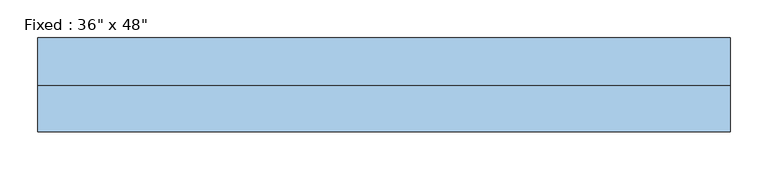
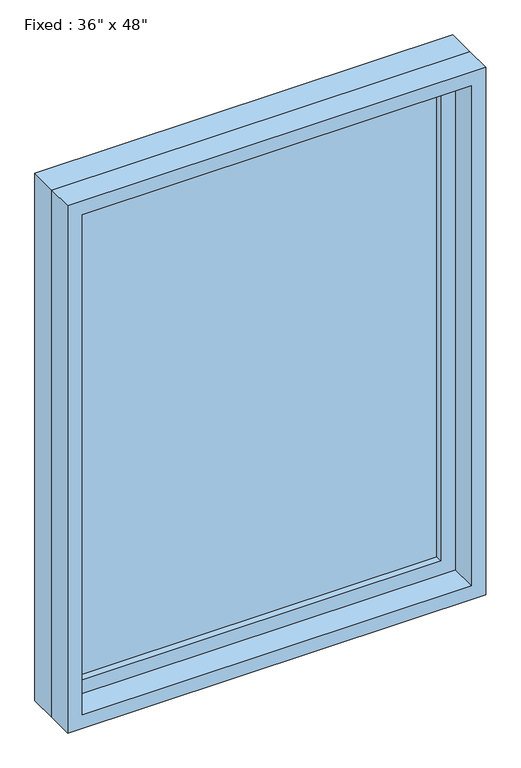
"""IFC4 building model written with IfcOpenShell, lengths in millimetres: window geometry."""

import ifcopenshell
import ifcopenshell.guid

model = None  # the IFC model being written
_history = None  # IfcOwnerHistory: only IFC2X3 demands one
_inside = {}  # id of a spatial element -> (the spatial element, [elements in it])
_under = {}  # id of a project, library or spatial element -> (it, [spatial elements below it])
_declared = {}  # id of a project -> (the project, [libraries it declares])
_typed = {}  # id of a type object -> (the type object, [elements of that type])
_made_of = {}  # id of a material, layer set ... -> (it, [elements and type objects made of it])


def new_model(schema):
    """Start an empty IFC model of exactly this schema.

    Asked for "IFC4X3", IfcOpenShell would pick the latest addendum, in which some entities
    have other attributes; the version numbers below select the first issue.
    IFC2X3 requires an IfcOwnerHistory on every rooted entity: one is made here for all.
    """
    global model, _history
    if schema == "IFC4X3":
        model = ifcopenshell.file(schema_version=(4, 3, 0, 0))
    else:
        model = ifcopenshell.file(schema=schema)
    _inside.clear()
    _under.clear()
    _declared.clear()
    _typed.clear()
    _made_of.clear()
    _history = None
    if model.schema == "IFC2X3":
        org = make("IfcOrganization", Name="unknown")
        user = make(
            "IfcPersonAndOrganization",
            ThePerson=make("IfcPerson", FamilyName="unknown"),
            TheOrganization=org,
        )
        app = make(
            "IfcApplication",
            ApplicationDeveloper=org,
            Version="unknown",
            ApplicationFullName="unknown",
            ApplicationIdentifier="unknown",
        )
        _history = make(
            "IfcOwnerHistory",
            OwningUser=user,
            OwningApplication=app,
            ChangeAction="ADDED",
            CreationDate=0,
        )
    return model


def make(cls, **values):
    """One entity of the class cls with the attributes given. An attribute that is None is left unset."""
    return model.create_entity(
        cls, **{name: value for name, value in values.items() if value is not None}
    )


def rooted(cls, **values):
    """An entity with a GlobalId (a new one), such as an element, a storey or a relation."""
    return make(cls, GlobalId=ifcopenshell.guid.new(), OwnerHistory=_history, **values)


def si_unit(unit_type, name, prefix=None):
    """IfcSIUnit, for example si_unit("LENGTHUNIT", "METRE", prefix="MILLI")."""
    return make("IfcSIUnit", UnitType=unit_type, Prefix=prefix, Name=name)


def assignment(units):
    """IfcUnitAssignment: the units of a project."""
    return None if units is None else make("IfcUnitAssignment", Units=units)


def point(xyz):
    """IfcCartesianPoint."""
    return None if xyz is None else make("IfcCartesianPoint", Coordinates=xyz)


def direction(xyz):
    """IfcDirection."""
    return None if xyz is None else make("IfcDirection", DirectionRatios=xyz)


def frame(location, z_axis=None, x_axis=None):
    """IfcAxis2Placement3D, a coordinate frame: its origin and axes. An axis left out is left unset."""
    return make(
        "IfcAxis2Placement3D",
        Location=point(location),
        Axis=direction(z_axis),
        RefDirection=direction(x_axis),
    )


def origin():
    """The frame at (0, 0, 0) with its axes left unset."""
    return frame((0.0, 0.0, 0.0))


def place(relative_to, where):
    """IfcLocalPlacement: puts the frame where relative to a parent placement (None: the world)."""
    return make(
        "IfcLocalPlacement", PlacementRelTo=relative_to, RelativePlacement=where
    )


def context(
    kind, dimensions, precision=None, world=None, true_north=None, identifier=None
):
    """IfcGeometricRepresentationContext, for example the 3D "Model" context."""
    return make(
        "IfcGeometricRepresentationContext",
        ContextIdentifier=identifier,
        ContextType=kind,
        CoordinateSpaceDimension=dimensions,
        Precision=precision,
        WorldCoordinateSystem=world,
        TrueNorth=true_north,
    )


def project(units=None, contexts=None):
    """IfcProject with its units and contexts."""
    return rooted(
        "IfcProject",
        Name="project",
        RepresentationContexts=contexts,
        UnitsInContext=assignment(units),
    )


def spatial(cls, under=None, at=None, **own):
    """A site, building, storey or space (cls), placed at a placement, below another one or the project."""
    s = rooted(cls, ObjectPlacement=at, **own)
    if under is not None:
        _under.setdefault(under.id(), (under, []))[1].append(s)
    return s


def polyline(points):
    """IfcPolyline through the points."""
    return make("IfcPolyline", Points=[point(p) for p in points])


def outline(outer, holes=None, kind="AREA"):
    """IfcArbitraryClosedProfileDef: a profile drawn as a closed curve; with holes, ...WithVoids."""
    if holes is None:
        return make("IfcArbitraryClosedProfileDef", ProfileType=kind, OuterCurve=outer)
    return make(
        "IfcArbitraryProfileDefWithVoids",
        ProfileType=kind,
        OuterCurve=outer,
        InnerCurves=holes,
    )


def extrude(swept, where, along, depth):
    """IfcExtrudedAreaSolid: the profile swept, set in the frame where, extruded along a direction by depth."""
    return make(
        "IfcExtrudedAreaSolid",
        SweptArea=swept,
        Position=where,
        ExtrudedDirection=direction(along),
        Depth=depth,
    )


def shape(context_of_items, identifier, shape_type, items):
    """IfcShapeRepresentation: the items that make up one representation, for example the "Body"."""
    return make(
        "IfcShapeRepresentation",
        ContextOfItems=context_of_items,
        RepresentationIdentifier=identifier,
        RepresentationType=shape_type,
        Items=items,
    )


def source(mapping_origin, context_of_items, identifier, shape_type, items):
    """IfcRepresentationMap: a shape defined once, which mapped items show again and again."""
    return make(
        "IfcRepresentationMap",
        MappingOrigin=mapping_origin,
        MappedRepresentation=shape(context_of_items, identifier, shape_type, items),
    )


def transform(
    local_origin,
    x_axis=None,
    y_axis=None,
    z_axis=None,
    scale=None,
    scale2=None,
    scale3=None,
    uniform=True,
):
    """IfcCartesianTransformationOperator3D, or its non-uniform kind. x_axis, y_axis, z_axis: its Axis1, 2, 3."""
    if uniform:
        return make(
            "IfcCartesianTransformationOperator3D",
            Axis1=direction(x_axis),
            Axis2=direction(y_axis),
            LocalOrigin=point(local_origin),
            Scale=scale,
            Axis3=direction(z_axis),
        )
    return make(
        "IfcCartesianTransformationOperator3DnonUniform",
        Axis1=direction(x_axis),
        Axis2=direction(y_axis),
        LocalOrigin=point(local_origin),
        Scale=scale,
        Axis3=direction(z_axis),
        Scale2=scale2,
        Scale3=scale3,
    )


def mapped(mapping_source, mapping_target):
    """IfcMappedItem: shows the shape of a source again, moved by a transform."""
    return make(
        "IfcMappedItem", MappingSource=mapping_source, MappingTarget=mapping_target
    )


def made_of(thing, what):
    """Note that an element or type object is made of a material, layer set ...; save() writes the relation."""
    if what is not None:
        _made_of.setdefault(what.id(), (what, []))[1].append(thing)
    return thing


def element(
    cls,
    number,
    at=None,
    inside=None,
    cuts=None,
    type_object=None,
    material=None,
    context=None,
    identifier="Body",
    shape_type=None,
    held_by="IfcProductDefinitionShape",
    body=None,
    shapes=None,
    **own,
):
    """One element of the class cls, such as IfcWall. Its Tag is "e" and its number.

    at: its placement. inside: the storey or other place that contains it. cuts: it is an
    opening in that element (IfcRelVoidsElement). A single representation is given by context,
    identifier, shape_type and body (its items); several are given by shapes. held_by: the class
    of the entity that holds the representations. save() writes the other relations.
    """
    e = rooted(cls, Tag="e%d" % number, ObjectPlacement=at, **own)
    if body is not None:
        shapes = [shape(context, identifier, shape_type, body)]
    if shapes is not None:
        e.Representation = make(held_by, Representations=shapes)
    if inside is not None:
        _inside.setdefault(inside.id(), (inside, []))[1].append(e)
    if cuts is not None:
        rooted(
            "IfcRelVoidsElement", RelatingBuildingElement=cuts, RelatedOpeningElement=e
        )
    if type_object is not None:
        _typed.setdefault(type_object.id(), (type_object, []))[1].append(e)
    return made_of(e, material)


def aggregate(whole, parts):
    """IfcRelAggregates: a whole, such as a stair, and the parts it consists of."""
    return rooted("IfcRelAggregates", RelatingObject=whole, RelatedObjects=parts)


def save(model, path):
    """Write the relations noted so far, then the file.

    IfcRelAggregates (storeys below a building ...), IfcRelContainedInSpatialStructure (elements
    in a storey), IfcRelDefinesByType, IfcRelAssociatesMaterial and IfcRelDeclares: one each for
    every whole, place, type object, material and project.
    """
    for whole, parts in _under.values():
        aggregate(whole, parts)
    for where, things in _inside.values():
        rooted(
            "IfcRelContainedInSpatialStructure",
            RelatedElements=things,
            RelatingStructure=where,
        )
    for kind, things in _typed.values():
        rooted("IfcRelDefinesByType", RelatedObjects=things, RelatingType=kind)
    for what, things in _made_of.values():
        rooted("IfcRelAssociatesMaterial", RelatedObjects=things, RelatingMaterial=what)
    for by, libraries in _declared.values():
        rooted("IfcRelDeclares", RelatingContext=by, RelatedDefinitions=libraries)
    model.write(path)


def window_96cf1632(model_context):
    return source(origin(), model_context, "Body", "SweptSolid", [
        extrude(outline(polyline([(355.6, 14.2875), (-431.8, 14.2875), (-431.8, 26.9875), (355.6, 26.9875), (355.6, 14.2875)])), frame((0.0, 0.0, 977.9), z_axis=(0.0, 0.0, 1.0), x_axis=(1.0, 0.0, 0.0)), (0.0, 0.0, 1.0), 1092.2),
        extrude(outline(polyline([(2114.55, -476.25), (933.45, -476.25), (933.45, 400.05), (2114.55, 400.05), (2114.55, -476.25)]), holes=[polyline([(2070.1, -431.8), (2070.1, 355.6), (977.9, 355.6), (977.9, -431.8), (2070.1, -431.8)])]), frame((0.0, -1.5875, 0.0), z_axis=(0.0, 1.0, 0.0), x_axis=(0.0, 0.0, 1.0)), (0.0, 0.0, 1.0), 44.45),
        extrude(outline(polyline([(2133.6, -495.3), (914.4, -495.3), (914.4, 419.1), (2133.6, 419.1), (2133.6, -495.3)]), holes=[polyline([(2101.85, -463.55), (2101.85, 387.35), (946.15, 387.35), (946.15, -463.55), (2101.85, -463.55)])]), frame((0.0, -61.9125, 0.0), z_axis=(0.0, 1.0, 0.0), x_axis=(0.0, 0.0, 1.0)), (0.0, 0.0, 1.0), 60.325),
        extrude(outline(polyline([(2133.6, 419.1), (2133.6, -495.3), (914.4, -495.3), (914.4, 419.1), (2133.6, 419.1)]), holes=[polyline([(2114.55, 400.05), (933.45, 400.05), (933.45, -476.25), (2114.55, -476.25), (2114.55, 400.05)])]), frame((0.0, -1.5875, 0.0), z_axis=(0.0, 1.0, 0.0), x_axis=(0.0, 0.0, 1.0)), (0.0, 0.0, 1.0), 63.5),
    ])


if __name__ == "__main__":
    model = new_model("IFC4")
    model_context = context("Model", 3, world=origin())
    ifc_project = project(units=[si_unit("LENGTHUNIT", "METRE", prefix="MILLI")], contexts=[model_context])
    site = spatial("IfcSite", under=ifc_project)
    building = spatial("IfcBuilding", under=site)
    placement = place(None, origin())
    window_shape = window_96cf1632(model_context)
    element("IfcWindow", 1, ObjectType="Fixed : 36\" x 48\"", at=placement, inside=building, context=model_context, shape_type="MappedRepresentation", body=[
        mapped(window_shape, transform((0.0, 0.0, 0.0), x_axis=(1.0, 0.0, 0.0), y_axis=(0.0, 1.0, 0.0), z_axis=(0.0, 0.0, 1.0))),
    ])
    save(model, "model.ifc")

# Revit data of these elements
# Type "Fixed : 36\" x 48\""
#   Type Mark = "1"
#   Assembly Code = "B2020100"
#   Height = 4' - 0"
#   Default Sill Height = 3' - 0"
#   Width = 3' - 0"
#   Window Inset = 0' - 0 3/4"
#   Glass Pane Material = Glass
#   Sash Material = Sash
#   Wall Closure = (empty or 0)
# Element 1 (IfcWindow, "Fixed : 36\" x 48\"")
#   Materials on its faces: "Sash", "Glass"
# Materials
#   "Glass": class "Glass", colour RGB 0 128 192, transparency 0.75
#   "Sash": class "Wood", colour RGB 224 178 126, transparency 0
